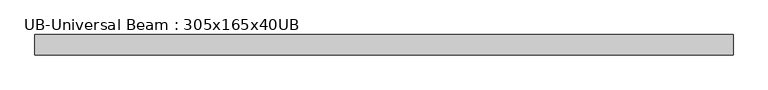
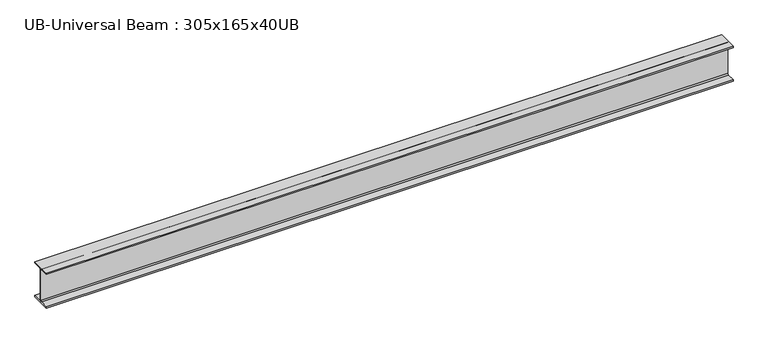
"""IFC4 building model written with IfcOpenShell, lengths in millimetres: beam geometry, UB-Universal Beam : 305x165x40UB."""

from ifc_helpers import new_model, si_unit, point, frame, frame_2d, origin, place, context, project, spatial, polyline, circle_curve, trimmed, segment, composite_curve, outline, extrude, source, transform, mapped, element, save


def ub_universal_beam_305x165x40ub_26306981(model_context):
    return source(origin(), model_context, "Body", "SweptSolid", [
        extrude(outline(composite_curve([segment(polyline([(82.5, -141.5), (82.5, -151.7), (-82.5, -151.7), (-82.5, -141.5), (-11.9, -141.5)]), True, "CONTINUOUS"), segment(trimmed(circle_curve(frame_2d((-11.9, -132.6)), 8.9), [point((-11.9, -141.5))], [point((-3.0, -132.6))], True, "CARTESIAN"), True, "CONTINUOUS"), segment(polyline([(-3.0, -132.6), (-3.0, 132.6)]), True, "CONTINUOUS"), segment(trimmed(circle_curve(frame_2d((-11.9, 132.6)), 8.9), [point((-3.0, 132.6))], [point((-11.9, 141.5))], True, "CARTESIAN"), True, "CONTINUOUS"), segment(polyline([(-11.9, 141.5), (-82.5, 141.5), (-82.5, 151.7), (82.5, 151.7), (82.5, 141.5), (11.9, 141.5)]), True, "CONTINUOUS"), segment(trimmed(circle_curve(frame_2d((11.9, 132.6)), 8.9), [point((11.9, 141.5))], [point((3.0, 132.6))], True, "CARTESIAN"), True, "CONTINUOUS"), segment(polyline([(3.0, 132.6), (3.0, -132.6)]), True, "CONTINUOUS"), segment(trimmed(circle_curve(frame_2d((11.9, -132.6)), 8.9), [point((3.0, -132.6))], [point((11.9, -141.5))], True, "CARTESIAN"), True, "CONTINUOUS"), segment(polyline([(11.9, -141.5), (82.5, -141.5)]), True, "CONTINUOUS")], self_intersect=False)), frame((-2832.175, 0.0, 0.0), z_axis=(1.0, 0.0, 0.0), x_axis=(0.0, 1.0, 0.0)), (0.0, 0.0, 1.0), 5664.35),
    ])


if __name__ == "__main__":
    model = new_model("IFC4")
    model_context = context("Model", 3, world=origin())
    ifc_project = project(units=[si_unit("LENGTHUNIT", "METRE", prefix="MILLI")], contexts=[model_context])
    site = spatial("IfcSite", under=ifc_project)
    building = spatial("IfcBuilding", under=site)
    placement = place(None, origin())
    ub_universal_beam_305x165x40ub_shape = ub_universal_beam_305x165x40ub_26306981(model_context)
    element("IfcBeam", 1, ObjectType="UB-Universal Beam : 305x165x40UB", at=placement, inside=building, context=model_context, shape_type="MappedRepresentation", body=[
        mapped(ub_universal_beam_305x165x40ub_shape, transform((0.0, 0.0, 0.0), x_axis=(1.0, 0.0, 0.0), y_axis=(0.0, 1.0, 0.0), z_axis=(0.0, 0.0, 1.0))),
    ])
    save(model, "model.ifc")

# Revit data of these elements
# Type "UB-Universal Beam : 305x165x40UB"
#   Nominal h = "305"
#   W = 0
#   Start Extension Calculation [instance default] = 3000 mm
#   Start Extension [instance default] = -12.7 mm
#   End Extension Calculation [instance default] = 3000 mm
#   End Extension [instance default] = -12.7 mm
#   Ix = 8503
#   Length [instance default] = 1524 mm
#   M = 40.3
#   Zx = 560
#   b = 165 mm
#   h = 303.4 mm
#   r = 8.9 mm
#   s = 6 mm
#   t = 10.2 mm
#   A = 0.005 m²
#   Structural Material [instance default] = Metal - Steel - 345 MPa
#   Assembly Code = ""
# Element 1 (IfcBeam, "UB-Universal Beam : 305x165x40UB")
#   Materials on its faces: "Metal - Steel - 345 MPa"
# Materials
#   "Metal - Steel - 345 MPa": class "Metal", colour RGB 241 46 46, transparency 0
